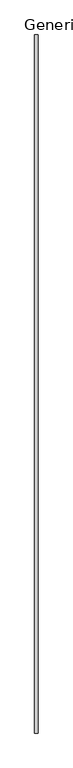
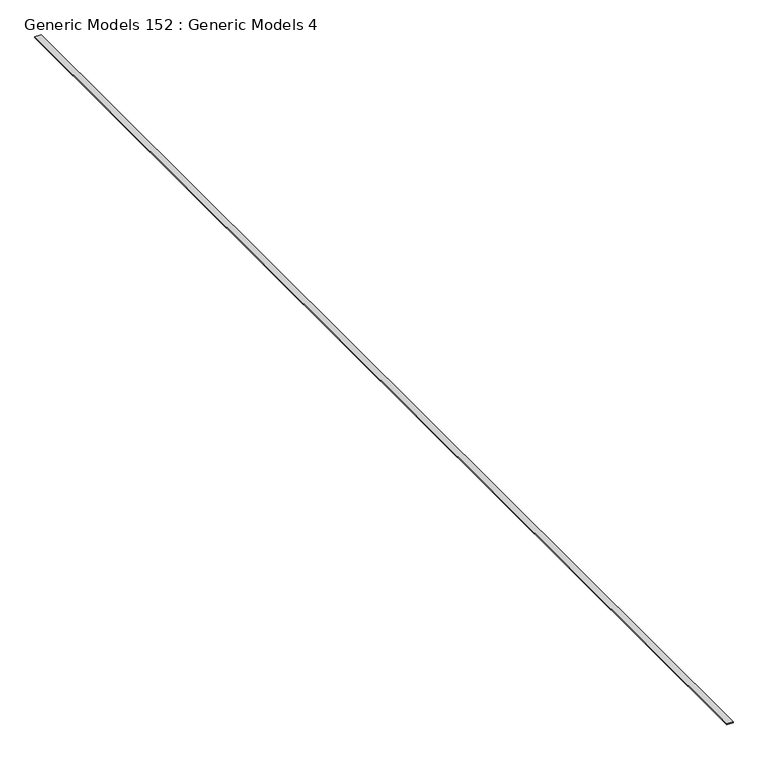
"""IFC4 building model written with IfcOpenShell, lengths in millimetres: proxy geometry, Generic Models 152 : Generic Models 4."""

from ifc_helpers import new_model, si_unit, frame, origin, place, context, project, spatial, polyline, outline, extrude, source, transform, mapped, element, save


def generic_models_152_generic_models_4_4f3bc147(model_context):
    return source(origin(), model_context, "Body", "SweptSolid", [
        extrude(outline(polyline([(-6524.9894166, -6864.9230338), (-6595.79305, -6864.9230338), (-6595.79305, 7054.2769662), (-6524.9894166, 7054.2769662), (-6524.9894166, -6864.9230338)])), frame((0.0, 0.0, 126183.5628287), z_axis=(0.0, 0.0, 1.0), x_axis=(1.0, 0.0, 0.0)), (0.0, 0.0, 1.0), 10.795),
    ])


if __name__ == "__main__":
    model = new_model("IFC4")
    model_context = context("Model", 3, world=origin())
    ifc_project = project(units=[si_unit("LENGTHUNIT", "METRE", prefix="MILLI")], contexts=[model_context])
    site = spatial("IfcSite", under=ifc_project)
    building = spatial("IfcBuilding", under=site)
    placement = place(None, origin())
    generic_models_152_generic_models_4_shape = generic_models_152_generic_models_4_4f3bc147(model_context)
    element("IfcBuildingElementProxy", 1, Name="Generic Models 152 : Generic Models 4", ObjectType="Generic Models 152 : Generic Models 4", at=placement, inside=building, context=model_context, shape_type="MappedRepresentation", body=[
        mapped(generic_models_152_generic_models_4_shape, transform((0.0, 0.0, 0.0), x_axis=(1.0, 0.0, 0.0), y_axis=(0.0, 1.0, 0.0), z_axis=(0.0, 0.0, 1.0))),
    ])
    save(model, "model.ifc")

# Revit data of these elements
# Element 1 (IfcBuildingElementProxy, "Generic Models 152 : Generic Models 4")
#   Materials on its faces: "_BLOCKING AS REQUIRED"
# Materials
#   "_BLOCKING AS REQUIRED": class "Generic", colour RGB 177 130 114, transparency 0, Cost = 0
